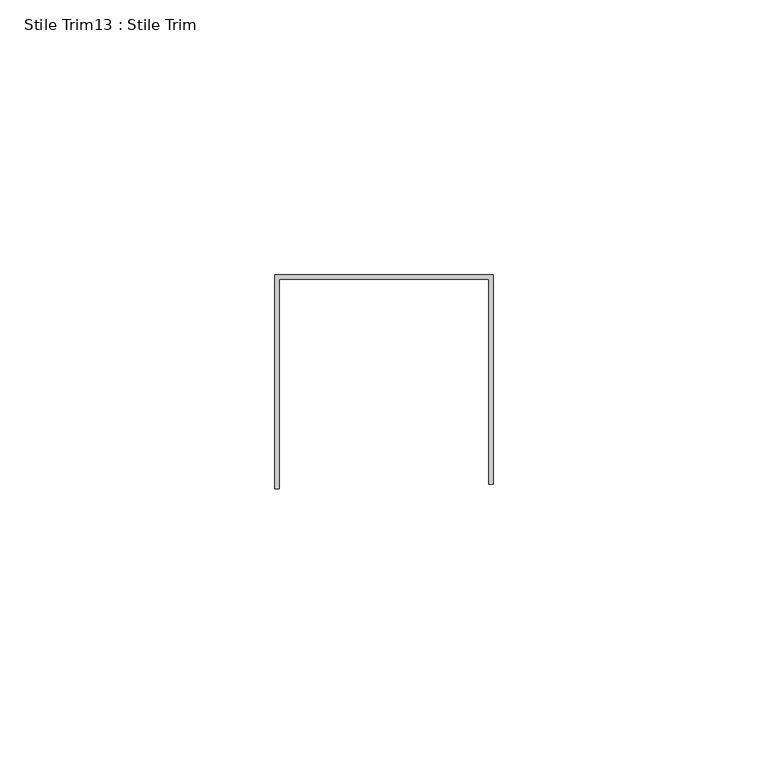
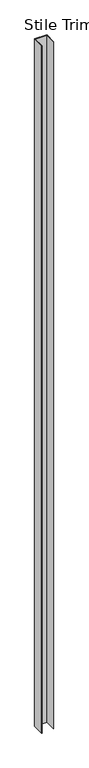
"""IFC4 building model written with IfcOpenShell, lengths in millimetres: proxy geometry, Stile Trim13 : Stile Trim."""

from ifc_helpers import new_model, si_unit, frame, origin, place, context, project, spatial, polyline, outline, extrude, source, transform, mapped, element, save


def stile_trim13_stile_trim_02668cd7(model_context):
    return source(origin(), model_context, "Body", "SweptSolid", [
        extrude(outline(polyline([(587327.0060739, -531784.4789841), (587366.6808739, -531784.4789841), (587366.6808739, -531822.5789841), (587365.8934739, -531822.5789841), (587365.8934739, -531785.2663841), (587327.7934739, -531785.2663841), (587327.7934739, -531823.3663841), (587327.0060739, -531823.3663841), (587327.0060739, -531784.4789841)])), frame((0.0, 0.0, 50.8), z_axis=(0.0, 0.0, 1.0), x_axis=(1.0, 0.0, 0.0)), (0.0, 0.0, 1.0), 2350.3929688),
    ])


if __name__ == "__main__":
    model = new_model("IFC4")
    model_context = context("Model", 3, world=origin())
    ifc_project = project(units=[si_unit("LENGTHUNIT", "METRE", prefix="MILLI")], contexts=[model_context])
    site = spatial("IfcSite", under=ifc_project)
    building = spatial("IfcBuilding", under=site)
    placement = place(None, origin())
    stile_trim13_stile_trim_shape = stile_trim13_stile_trim_02668cd7(model_context)
    element("IfcBuildingElementProxy", 1, Name="Stile Trim13 : Stile Trim", ObjectType="Stile Trim13 : Stile Trim", at=placement, inside=building, context=model_context, shape_type="MappedRepresentation", body=[
        mapped(stile_trim13_stile_trim_shape, transform((0.0, 0.0, 0.0), x_axis=(1.0, 0.0, 0.0), y_axis=(0.0, 1.0, 0.0), z_axis=(0.0, 0.0, 1.0))),
    ])
    save(model, "model.ifc")

# Revit data of these elements
# Element 1 (IfcBuildingElementProxy, "Stile Trim13 : Stile Trim")
#   Materials on its faces: "EDGE TRIM BY MTL PANEL MFR."
# Materials
#   "EDGE TRIM BY MTL PANEL MFR.": class "Generic", colour RGB 239 242 240, transparency 0, Cost = 0
